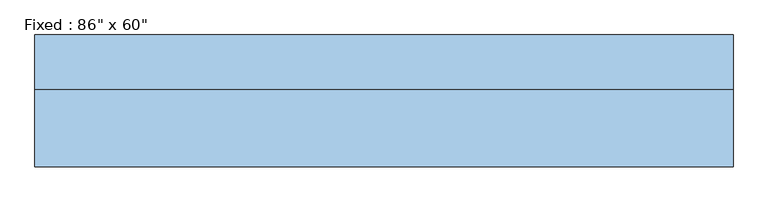
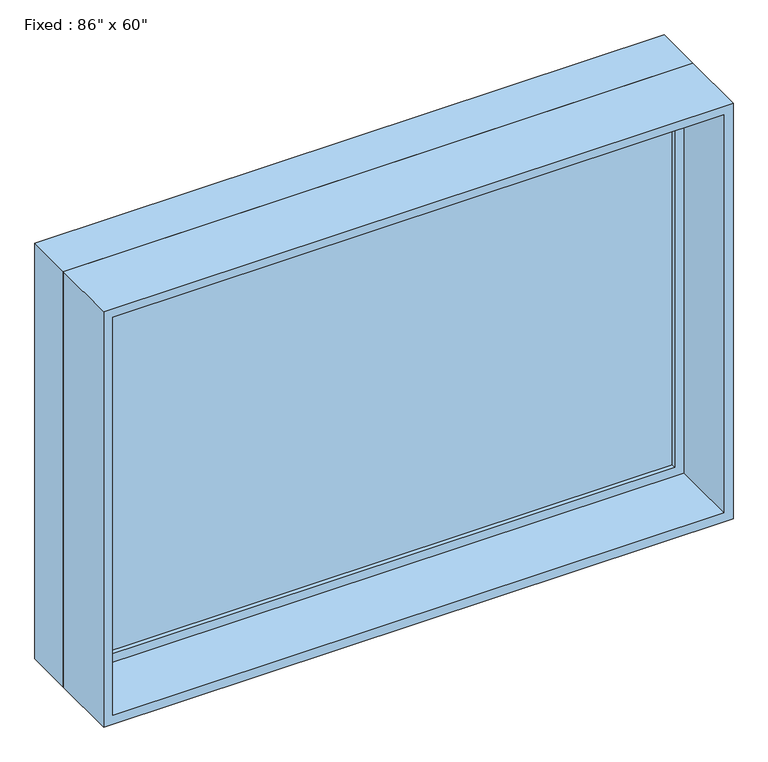
"""IFC4 building model written with IfcOpenShell, lengths in millimetres: window geometry."""

from ifc_helpers import new_model, si_unit, frame, origin, place, context, project, spatial, polyline, outline, extrude, source, transform, mapped, element, save


def window_d56d71bd(model_context):
    return source(origin(), model_context, "Body", "SweptSolid", [
        extrude(outline(polyline([(990.6, 50.8), (-1066.8, 50.8), (-1066.8, 63.5), (990.6, 63.5), (990.6, 50.8)])), frame((0.0, 0.0, 977.9), z_axis=(0.0, 0.0, 1.0), x_axis=(1.0, 0.0, 0.0)), (0.0, 0.0, 1.0), 1397.0),
        extrude(outline(polyline([(2419.35, -1111.25), (933.45, -1111.25), (933.45, 1035.05), (2419.35, 1035.05), (2419.35, -1111.25)]), holes=[polyline([(2374.9, -1066.8), (2374.9, 990.6), (977.9, 990.6), (977.9, -1066.8), (2374.9, -1066.8)])]), frame((0.0, 34.925, 0.0), z_axis=(0.0, 1.0, 0.0), x_axis=(0.0, 0.0, 1.0)), (0.0, 0.0, 1.0), 44.45),
        extrude(outline(polyline([(2438.4, -1130.3), (914.4, -1130.3), (914.4, 1054.1), (2438.4, 1054.1), (2438.4, -1130.3)]), holes=[polyline([(2406.65, -1098.55), (2406.65, 1022.35), (946.15, 1022.35), (946.15, -1098.55), (2406.65, -1098.55)])]), frame((0.0, -206.375, 0.0), z_axis=(0.0, 1.0, 0.0), x_axis=(0.0, 0.0, 1.0)), (0.0, 0.0, 1.0), 241.3),
        extrude(outline(polyline([(2438.4, 1054.1), (2438.4, -1130.3), (914.4, -1130.3), (914.4, 1054.1), (2438.4, 1054.1)]), holes=[polyline([(2419.35, 1035.05), (933.45, 1035.05), (933.45, -1111.25), (2419.35, -1111.25), (2419.35, 1035.05)])]), frame((0.0, 34.925, 0.0), z_axis=(0.0, 1.0, 0.0), x_axis=(0.0, 0.0, 1.0)), (0.0, 0.0, 1.0), 171.45),
    ])


if __name__ == "__main__":
    model = new_model("IFC4")
    model_context = context("Model", 3, world=origin())
    ifc_project = project(units=[si_unit("LENGTHUNIT", "METRE", prefix="MILLI")], contexts=[model_context])
    site = spatial("IfcSite", under=ifc_project)
    building = spatial("IfcBuilding", under=site)
    placement = place(None, origin())
    window_shape = window_d56d71bd(model_context)
    element("IfcWindow", 1, ObjectType="Fixed : 86\" x 60\"", at=placement, inside=building, context=model_context, shape_type="MappedRepresentation", body=[
        mapped(window_shape, transform((0.0, 0.0, 0.0), x_axis=(1.0, 0.0, 0.0), y_axis=(0.0, 1.0, 0.0), z_axis=(0.0, 0.0, 1.0))),
    ])
    save(model, "model.ifc")

# Revit data of these elements
# Type "Fixed : 86\" x 60\""
#   Type Mark = "19"
#   Construction Type Id = "GSP4R"
#   Assembly Code = "B2020100"
#   Analytic Construction = "1/8 in Pilkington single glazing"
#   Visual Light Transmittance = 0.9
#   Solar Heat Gain Coefficient = 0.78
#   Heat Transfer Coefficient (U) = 3.6886 W/(m²·K)
#   Height = 5' - 0"
#   Default Sill Height = 3' - 0"
#   Width = 7' - 2"
#   Window Inset = 0' - 5"
#   Glass Pane Material = Glass
#   Sash Material = Sash
#   Wall Closure = (empty or 0)
# Element 1 (IfcWindow, "Fixed : 86\" x 60\"")
#   Materials on its faces: "Sash", "Glass"
# Materials
#   "Glass": class "Glass", colour RGB 0 128 192, transparency 0.75, Description = "Soda Lime Glass", Cost = 0
#   "Sash": class "Wood", colour RGB 224 178 126, transparency 0
